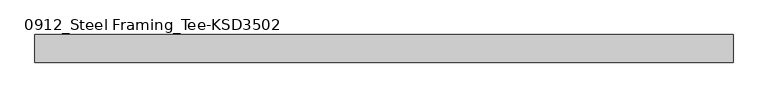
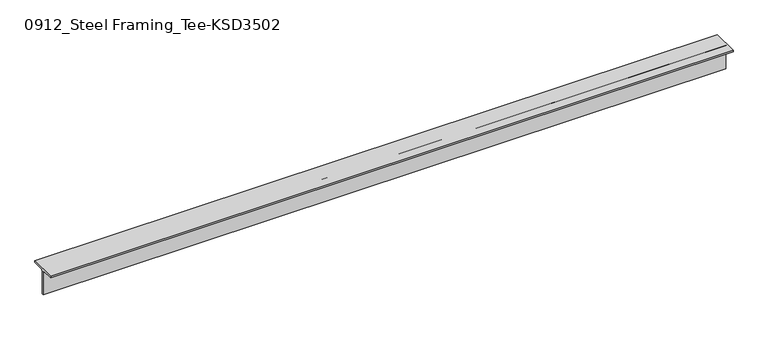
"""IFC4 building model written with IfcOpenShell, lengths in millimetres: member geometry, 0912_Steel Framing_Tee-KSD3502 : H_SB_ASB_CT-150x150x6.5x9."""

from ifc_helpers import new_model, si_unit, point, frame, frame_2d, origin, place, context, project, spatial, polyline, circle_curve, trimmed, segment, composite_curve, outline, extrude, source, transform, mapped, element, save


def member_0912_steel_framing_tee_ksd3502_2129ea9d(model_context):
    return source(origin(), model_context, "Body", "SweptSolid", [
        extrude(outline(composite_curve([segment(polyline([(-75.0, 75.0), (75.0, 75.0), (75.0, 66.0), (16.25, 66.0)]), True, "CONTINUOUS"), segment(trimmed(circle_curve(frame_2d((16.25, 53.0)), 13.0), [point((16.25, 66.0))], [point((3.25, 53.0))], True, "CARTESIAN"), True, "CONTINUOUS"), segment(polyline([(3.25, 53.0), (3.25, -75.0), (-3.25, -75.0), (-3.25, 53.0)]), True, "CONTINUOUS"), segment(trimmed(circle_curve(frame_2d((-16.25, 53.0)), 13.0), [point((-3.25, 53.0))], [point((-16.25, 66.0))], True, "CARTESIAN"), True, "CONTINUOUS"), segment(polyline([(-16.25, 66.0), (-75.0, 66.0), (-75.0, 75.0)]), True, "CONTINUOUS")], self_intersect=False)), frame((-1887.85, 0.0, 0.0), z_axis=(1.0, 0.0, 0.0), x_axis=(0.0, 1.0, 0.0)), (0.0, 0.0, 1.0), 3789.1),
    ])


if __name__ == "__main__":
    model = new_model("IFC4")
    model_context = context("Model", 3, world=origin())
    ifc_project = project(units=[si_unit("LENGTHUNIT", "METRE", prefix="MILLI")], contexts=[model_context])
    site = spatial("IfcSite", under=ifc_project)
    building = spatial("IfcBuilding", under=site)
    placement = place(None, origin())
    member_0912_steel_framing_tee_ksd3502_shape = member_0912_steel_framing_tee_ksd3502_2129ea9d(model_context)
    element("IfcMember", 1, ObjectType="0912_Steel Framing_Tee-KSD3502 : H_SB_ASB_CT-150x150x6.5x9", at=placement, inside=building, context=model_context, shape_type="MappedRepresentation", body=[
        mapped(member_0912_steel_framing_tee_ksd3502_shape, transform((0.0, 0.0, 0.0), x_axis=(1.0, 0.0, 0.0), y_axis=(0.0, 1.0, 0.0), z_axis=(0.0, 0.0, 1.0))),
    ])
    save(model, "model.ifc")

# Revit data of these elements
# Type "0912_Steel Framing_Tee-KSD3502 : H_SB_ASB_CT-150x150x6.5x9"
#   H_WM Code_1 = "S01AA003-00001 | Main Steel Structure Fabrication Work | Shelter/Building | Light Steel - Standard (30KG/M>Weight) | Material: (   )"
#   H_WM Code_2 = "S03AA029-00001 | Main Steel Structure Erection Work | Shelter/Building | Light Steel (30KG/M>Weight) | Material: (   )"
#   H_WM Code_3 = "S01AA010-00001 | Main Steel Structure Fabrication Work | Shelter/Building | Steel Painting/Coating | for Non-Fireproofed Steel Surface, Surface Preparation, Primer, Second & Final Coat | Material: (   )"
#   H_Q'ty Cal Type Tag = "SB-Q2"
#   Width = 15.0 cm
#   Web Thickness = 0.65 cm
#   Web Fillet = 1.3 cm
#   Section Area = 23.39 cm²
#   Perimeter = 0.60 m²/m
#   Nominal Weight = 18.40 kgf/m
#   Height = 15.0 cm
#   Flange Thickness = 0.9 cm
#   Centroid Vertical = 7.5 cm
#   Centroid Horizontal = 7.5 cm
#   Length [instance default] = 1.5000 m
#   Structural Material [instance default] = Steel, 45-345
#   Warping Constant = (empty or 0)
#   Torsional Moment of Inertia = 0
#   Section Name Key = ""
#   Plastic Modulus weak axis = 0
#   Plastic Modulus strong axis = 0
#   Moment of Inertia weak axis = 0
#   Moment of Inertia strong axis = 0
#   Elastic Modulus weak axis = 0
#   Elastic Modulus strong axis = 0
#   Bolt Spacing = 0
#   Assembly Code = ""
# Element 1 (IfcMember, "0912_Steel Framing_Tee-KSD3502 : H_SB_ASB_CT-150x150x6.5x9")
#   Structural Material = none
# Materials
#   "Steel, 45-345": class "Metal", colour RGB 189 187 185, transparency 0, Description = "Steel 345 MPa", Cost = 0
